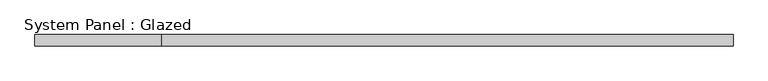
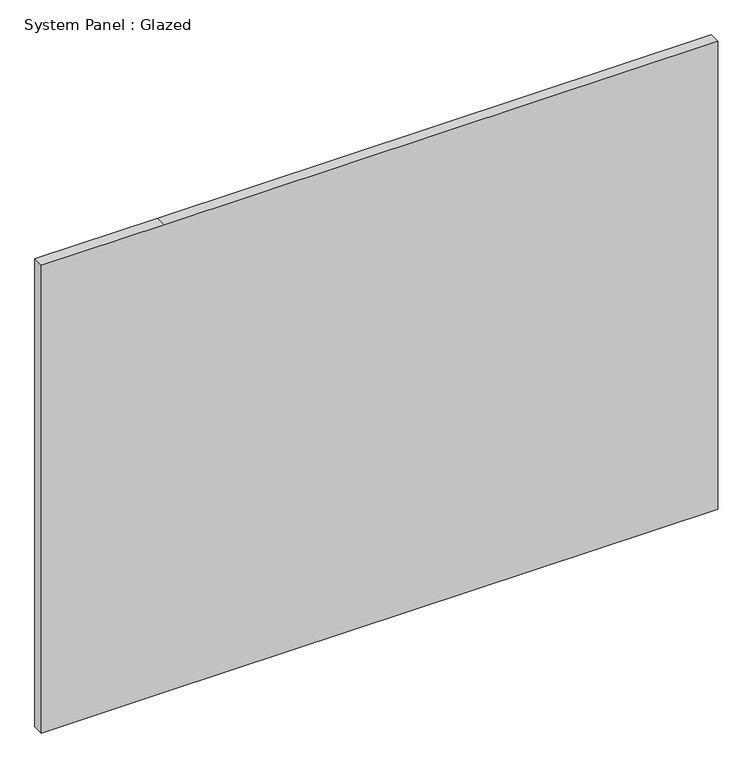
"""IFC4 building model written with IfcOpenShell, lengths in millimetres: plate geometry, System Panel : Glazed."""

from ifc_helpers import new_model, si_unit, frame, origin, place, context, project, spatial, polyline, outline, extrude, source, transform, mapped, element, save


def system_panel_glazed_639f3d85(model_context):
    return source(origin(), model_context, "Body", "SweptSolid", [
        extrude(outline(polyline([(0.0, -768.35), (0.0, -488.95), (0.0, 768.35), (1123.95, 768.35), (1123.95, -488.95), (1123.95, -768.35), (0.0, -768.35)])), frame((0.0, -44.45, 0.0), z_axis=(0.0, 1.0, 0.0), x_axis=(0.0, 0.0, 1.0)), (0.0, 0.0, 1.0), 25.4),
    ])


if __name__ == "__main__":
    model = new_model("IFC4")
    model_context = context("Model", 3, world=origin())
    ifc_project = project(units=[si_unit("LENGTHUNIT", "METRE", prefix="MILLI")], contexts=[model_context])
    site = spatial("IfcSite", under=ifc_project)
    building = spatial("IfcBuilding", under=site)
    placement = place(None, origin())
    system_panel_glazed_shape = system_panel_glazed_639f3d85(model_context)
    element("IfcPlate", 1, ObjectType="System Panel : Glazed", at=placement, inside=building, context=model_context, shape_type="MappedRepresentation", body=[
        mapped(system_panel_glazed_shape, transform((0.0, 0.0, 0.0), x_axis=(1.0, 0.0, 0.0), y_axis=(0.0, 1.0, 0.0), z_axis=(0.0, 0.0, 1.0))),
    ])
    save(model, "model.ifc")

# Revit data of these elements
# Element 1 (IfcPlate, "System Panel : Glazed")
#   Materials on its faces: "Glass"
# Materials
#   "Glass": class "Glass", colour RGB 0 128 192, transparency 0.75
